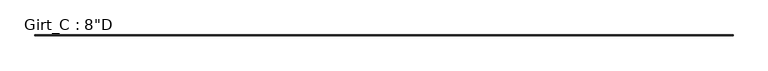
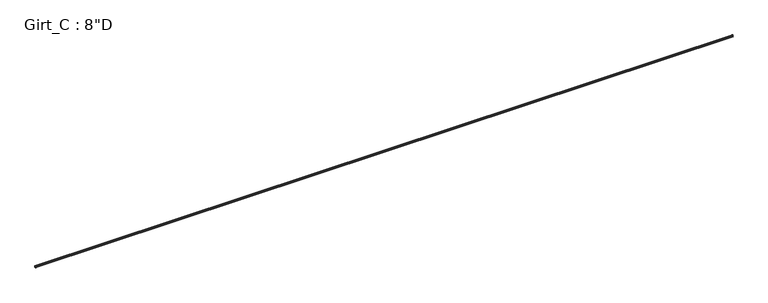
"""IFC4 building model written with IfcOpenShell, lengths in millimetres: beam geometry."""

import ifcopenshell
import ifcopenshell.guid

model = None  # the IFC model being written
_history = None  # IfcOwnerHistory: only IFC2X3 demands one
_inside = {}  # id of a spatial element -> (the spatial element, [elements in it])
_under = {}  # id of a project, library or spatial element -> (it, [spatial elements below it])
_declared = {}  # id of a project -> (the project, [libraries it declares])
_typed = {}  # id of a type object -> (the type object, [elements of that type])
_made_of = {}  # id of a material, layer set ... -> (it, [elements and type objects made of it])


def new_model(schema):
    """Start an empty IFC model of exactly this schema.

    Asked for "IFC4X3", IfcOpenShell would pick the latest addendum, in which some entities
    have other attributes; the version numbers below select the first issue.
    IFC2X3 requires an IfcOwnerHistory on every rooted entity: one is made here for all.
    """
    global model, _history
    if schema == "IFC4X3":
        model = ifcopenshell.file(schema_version=(4, 3, 0, 0))
    else:
        model = ifcopenshell.file(schema=schema)
    _inside.clear()
    _under.clear()
    _declared.clear()
    _typed.clear()
    _made_of.clear()
    _history = None
    if model.schema == "IFC2X3":
        org = make("IfcOrganization", Name="unknown")
        user = make(
            "IfcPersonAndOrganization",
            ThePerson=make("IfcPerson", FamilyName="unknown"),
            TheOrganization=org,
        )
        app = make(
            "IfcApplication",
            ApplicationDeveloper=org,
            Version="unknown",
            ApplicationFullName="unknown",
            ApplicationIdentifier="unknown",
        )
        _history = make(
            "IfcOwnerHistory",
            OwningUser=user,
            OwningApplication=app,
            ChangeAction="ADDED",
            CreationDate=0,
        )
    return model


def make(cls, **values):
    """One entity of the class cls with the attributes given. An attribute that is None is left unset."""
    return model.create_entity(
        cls, **{name: value for name, value in values.items() if value is not None}
    )


def rooted(cls, **values):
    """An entity with a GlobalId (a new one), such as an element, a storey or a relation."""
    return make(cls, GlobalId=ifcopenshell.guid.new(), OwnerHistory=_history, **values)


def si_unit(unit_type, name, prefix=None):
    """IfcSIUnit, for example si_unit("LENGTHUNIT", "METRE", prefix="MILLI")."""
    return make("IfcSIUnit", UnitType=unit_type, Prefix=prefix, Name=name)


def assignment(units):
    """IfcUnitAssignment: the units of a project."""
    return None if units is None else make("IfcUnitAssignment", Units=units)


def point(xyz):
    """IfcCartesianPoint."""
    return None if xyz is None else make("IfcCartesianPoint", Coordinates=xyz)


def direction(xyz):
    """IfcDirection."""
    return None if xyz is None else make("IfcDirection", DirectionRatios=xyz)


def frame(location, z_axis=None, x_axis=None):
    """IfcAxis2Placement3D, a coordinate frame: its origin and axes. An axis left out is left unset."""
    return make(
        "IfcAxis2Placement3D",
        Location=point(location),
        Axis=direction(z_axis),
        RefDirection=direction(x_axis),
    )


def frame_2d(location, x_axis=None):
    """IfcAxis2Placement2D, a coordinate frame in the plane: its origin and x axis."""
    return make(
        "IfcAxis2Placement2D", Location=point(location), RefDirection=direction(x_axis)
    )


def origin():
    """The frame at (0, 0, 0) with its axes left unset."""
    return frame((0.0, 0.0, 0.0))


def place(relative_to, where):
    """IfcLocalPlacement: puts the frame where relative to a parent placement (None: the world)."""
    return make(
        "IfcLocalPlacement", PlacementRelTo=relative_to, RelativePlacement=where
    )


def context(
    kind, dimensions, precision=None, world=None, true_north=None, identifier=None
):
    """IfcGeometricRepresentationContext, for example the 3D "Model" context."""
    return make(
        "IfcGeometricRepresentationContext",
        ContextIdentifier=identifier,
        ContextType=kind,
        CoordinateSpaceDimension=dimensions,
        Precision=precision,
        WorldCoordinateSystem=world,
        TrueNorth=true_north,
    )


def project(units=None, contexts=None):
    """IfcProject with its units and contexts."""
    return rooted(
        "IfcProject",
        Name="project",
        RepresentationContexts=contexts,
        UnitsInContext=assignment(units),
    )


def spatial(cls, under=None, at=None, **own):
    """A site, building, storey or space (cls), placed at a placement, below another one or the project."""
    s = rooted(cls, ObjectPlacement=at, **own)
    if under is not None:
        _under.setdefault(under.id(), (under, []))[1].append(s)
    return s


def polyline(points):
    """IfcPolyline through the points."""
    return make("IfcPolyline", Points=[point(p) for p in points])


def circle_curve(where, radius):
    """IfcCircle in the frame where."""
    return make("IfcCircle", Position=where, Radius=radius)


def trimmed(basis, trim1, trim2, sense, master):
    """IfcTrimmedCurve: the piece of a basis curve between two trims."""
    return make(
        "IfcTrimmedCurve",
        BasisCurve=basis,
        Trim1=trim1,
        Trim2=trim2,
        SenseAgreement=sense,
        MasterRepresentation=master,
    )


def segment(curve, same_sense, transition):
    """IfcCompositeCurveSegment."""
    return make(
        "IfcCompositeCurveSegment",
        Transition=transition,
        SameSense=same_sense,
        ParentCurve=curve,
    )


def composite_curve(segments, self_intersect=None):
    """IfcCompositeCurve: segments joined end to end."""
    return make("IfcCompositeCurve", Segments=segments, SelfIntersect=self_intersect)


def outline(outer, holes=None, kind="AREA"):
    """IfcArbitraryClosedProfileDef: a profile drawn as a closed curve; with holes, ...WithVoids."""
    if holes is None:
        return make("IfcArbitraryClosedProfileDef", ProfileType=kind, OuterCurve=outer)
    return make(
        "IfcArbitraryProfileDefWithVoids",
        ProfileType=kind,
        OuterCurve=outer,
        InnerCurves=holes,
    )


def extrude(swept, where, along, depth):
    """IfcExtrudedAreaSolid: the profile swept, set in the frame where, extruded along a direction by depth."""
    return make(
        "IfcExtrudedAreaSolid",
        SweptArea=swept,
        Position=where,
        ExtrudedDirection=direction(along),
        Depth=depth,
    )


def shape(context_of_items, identifier, shape_type, items):
    """IfcShapeRepresentation: the items that make up one representation, for example the "Body"."""
    return make(
        "IfcShapeRepresentation",
        ContextOfItems=context_of_items,
        RepresentationIdentifier=identifier,
        RepresentationType=shape_type,
        Items=items,
    )


def source(mapping_origin, context_of_items, identifier, shape_type, items):
    """IfcRepresentationMap: a shape defined once, which mapped items show again and again."""
    return make(
        "IfcRepresentationMap",
        MappingOrigin=mapping_origin,
        MappedRepresentation=shape(context_of_items, identifier, shape_type, items),
    )


def transform(
    local_origin,
    x_axis=None,
    y_axis=None,
    z_axis=None,
    scale=None,
    scale2=None,
    scale3=None,
    uniform=True,
):
    """IfcCartesianTransformationOperator3D, or its non-uniform kind. x_axis, y_axis, z_axis: its Axis1, 2, 3."""
    if uniform:
        return make(
            "IfcCartesianTransformationOperator3D",
            Axis1=direction(x_axis),
            Axis2=direction(y_axis),
            LocalOrigin=point(local_origin),
            Scale=scale,
            Axis3=direction(z_axis),
        )
    return make(
        "IfcCartesianTransformationOperator3DnonUniform",
        Axis1=direction(x_axis),
        Axis2=direction(y_axis),
        LocalOrigin=point(local_origin),
        Scale=scale,
        Axis3=direction(z_axis),
        Scale2=scale2,
        Scale3=scale3,
    )


def mapped(mapping_source, mapping_target):
    """IfcMappedItem: shows the shape of a source again, moved by a transform."""
    return make(
        "IfcMappedItem", MappingSource=mapping_source, MappingTarget=mapping_target
    )


def made_of(thing, what):
    """Note that an element or type object is made of a material, layer set ...; save() writes the relation."""
    if what is not None:
        _made_of.setdefault(what.id(), (what, []))[1].append(thing)
    return thing


def element(
    cls,
    number,
    at=None,
    inside=None,
    cuts=None,
    type_object=None,
    material=None,
    context=None,
    identifier="Body",
    shape_type=None,
    held_by="IfcProductDefinitionShape",
    body=None,
    shapes=None,
    **own,
):
    """One element of the class cls, such as IfcWall. Its Tag is "e" and its number.

    at: its placement. inside: the storey or other place that contains it. cuts: it is an
    opening in that element (IfcRelVoidsElement). A single representation is given by context,
    identifier, shape_type and body (its items); several are given by shapes. held_by: the class
    of the entity that holds the representations. save() writes the other relations.
    """
    e = rooted(cls, Tag="e%d" % number, ObjectPlacement=at, **own)
    if body is not None:
        shapes = [shape(context, identifier, shape_type, body)]
    if shapes is not None:
        e.Representation = make(held_by, Representations=shapes)
    if inside is not None:
        _inside.setdefault(inside.id(), (inside, []))[1].append(e)
    if cuts is not None:
        rooted(
            "IfcRelVoidsElement", RelatingBuildingElement=cuts, RelatedOpeningElement=e
        )
    if type_object is not None:
        _typed.setdefault(type_object.id(), (type_object, []))[1].append(e)
    return made_of(e, material)


def aggregate(whole, parts):
    """IfcRelAggregates: a whole, such as a stair, and the parts it consists of."""
    return rooted("IfcRelAggregates", RelatingObject=whole, RelatedObjects=parts)


def save(model, path):
    """Write the relations noted so far, then the file.

    IfcRelAggregates (storeys below a building ...), IfcRelContainedInSpatialStructure (elements
    in a storey), IfcRelDefinesByType, IfcRelAssociatesMaterial and IfcRelDeclares: one each for
    every whole, place, type object, material and project.
    """
    for whole, parts in _under.values():
        aggregate(whole, parts)
    for where, things in _inside.values():
        rooted(
            "IfcRelContainedInSpatialStructure",
            RelatedElements=things,
            RelatingStructure=where,
        )
    for kind, things in _typed.values():
        rooted("IfcRelDefinesByType", RelatedObjects=things, RelatingType=kind)
    for what, things in _made_of.values():
        rooted("IfcRelAssociatesMaterial", RelatedObjects=things, RelatingMaterial=what)
    for by, libraries in _declared.values():
        rooted("IfcRelDeclares", RelatingContext=by, RelatedDefinitions=libraries)
    model.write(path)


def beam_8d9c0b98(model_context):
    return source(origin(), model_context, "Body", "SweptSolid", [
        extrude(outline(composite_curve([segment(polyline([(-87.5109375, 101.6), (-3.3734375, 101.6)]), True, "CONTINUOUS"), segment(trimmed(circle_curve(frame_2d((-3.3734375, 96.8375)), 4.7625), [point((-3.3734375, 101.6))], [point((1.3890625, 96.8375))], False, "CARTESIAN"), True, "CONTINUOUS"), segment(polyline([(1.3890625, 96.8375), (1.3890625, -96.8375)]), True, "CONTINUOUS"), segment(trimmed(circle_curve(frame_2d((-3.3734375, -96.8375)), 4.7625), [point((1.3890625, -96.8375))], [point((-3.3734375, -101.6))], False, "CARTESIAN"), True, "CONTINUOUS"), segment(polyline([(-3.3734375, -101.6), (-87.5109375, -101.6), (-99.7792647, -86.979177), (-97.6510975, -85.1934327), (-86.2154765, -98.821875), (-3.2694106, -98.821875)]), True, "CONTINUOUS"), segment(trimmed(circle_curve(frame_2d((-3.3748024, -96.8389339)), 1.9857399), [point((-3.2694106, -98.821875))], [point((-1.3890625, -96.8389339))], True, "CARTESIAN"), True, "CONTINUOUS"), segment(polyline([(-1.3890625, -96.8389339), (-1.3890625, 96.8381931)]), True, "CONTINUOUS"), segment(trimmed(circle_curve(frame_2d((-3.3741066, 96.8381931)), 1.9850441), [point((-1.3890625, 96.8381931))], [point((-3.3005807, 98.821875))], True, "CARTESIAN"), True, "CONTINUOUS"), segment(polyline([(-3.3005807, 98.821875), (-86.2154765, 98.821875), (-97.6278742, 85.221109), (-99.7560415, 87.0068534), (-87.5109375, 101.6)]), True, "CONTINUOUS")], self_intersect=False)), frame((-44450.0, 0.0, 0.0), z_axis=(1.0, 0.0, 0.0), x_axis=(0.0, 1.0, 0.0)), (0.0, 0.0, 1.0), 88900.0),
    ])


if __name__ == "__main__":
    model = new_model("IFC4")
    model_context = context("Model", 3, world=origin())
    ifc_project = project(units=[si_unit("LENGTHUNIT", "METRE", prefix="MILLI")], contexts=[model_context])
    site = spatial("IfcSite", under=ifc_project)
    building = spatial("IfcBuilding", under=site)
    placement = place(None, origin())
    beam_shape = beam_8d9c0b98(model_context)
    element("IfcBeam", 1, ObjectType="Girt_C : 8\"D", at=placement, inside=building, context=model_context, shape_type="MappedRepresentation", body=[
        mapped(beam_shape, transform((0.0, 0.0, 0.0), x_axis=(1.0, 0.0, 0.0), y_axis=(0.0, 1.0, 0.0), z_axis=(0.0, 0.0, 1.0))),
    ])
    save(model, "model.ifc")

# Revit data of these elements
# Type "Girt_C : 8\"D"
#   half leg = 0' - 1 3/4"
#   Web_Thickness = 0' - 0 7/64"
#   Length [instance default] = 10' - 0"
#   Leg_1 = 0' - 3 1/2"
#   Height = 0' - 8"
#   Structural Material [instance default] = none
# Element 1 (IfcBeam, "Girt_C : 8\"D")
#   Structural Material = CEE' SECTION (8.0x3.5C - SEE STRUCT. DWGS)
#   Materials on its faces: "CEE' SECTION (8.0x3.5C - SEE STRUCT. DWGS)"
# Materials
#   "CEE' SECTION (8.0x3.5C - SEE STRUCT. DWGS)": class "Metal", colour RGB 137 146 153, transparency 0, Description = "Steel, mill finish", Cost = 0
